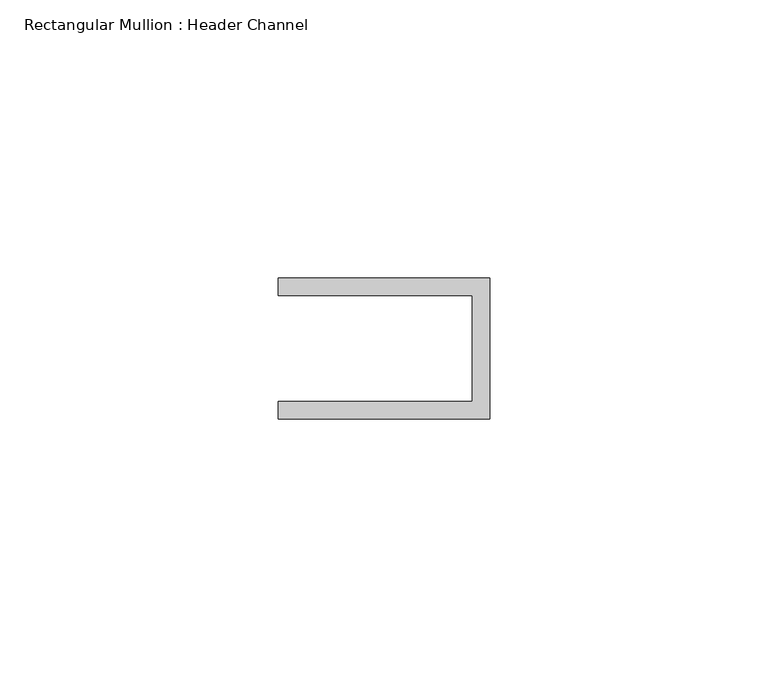
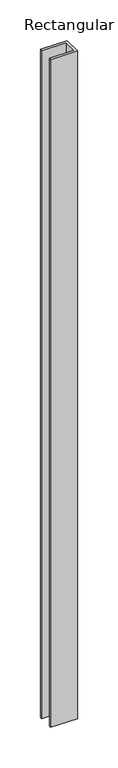
"""IFC4 building model written with IfcOpenShell, lengths in millimetres: member geometry, Rectangular Mullion : Header Channel."""

import ifcopenshell
import ifcopenshell.guid

model = None  # the IFC model being written
_history = None  # IfcOwnerHistory: only IFC2X3 demands one
_inside = {}  # id of a spatial element -> (the spatial element, [elements in it])
_under = {}  # id of a project, library or spatial element -> (it, [spatial elements below it])
_declared = {}  # id of a project -> (the project, [libraries it declares])
_typed = {}  # id of a type object -> (the type object, [elements of that type])
_made_of = {}  # id of a material, layer set ... -> (it, [elements and type objects made of it])


def new_model(schema):
    """Start an empty IFC model of exactly this schema.

    Asked for "IFC4X3", IfcOpenShell would pick the latest addendum, in which some entities
    have other attributes; the version numbers below select the first issue.
    IFC2X3 requires an IfcOwnerHistory on every rooted entity: one is made here for all.
    """
    global model, _history
    if schema == "IFC4X3":
        model = ifcopenshell.file(schema_version=(4, 3, 0, 0))
    else:
        model = ifcopenshell.file(schema=schema)
    _inside.clear()
    _under.clear()
    _declared.clear()
    _typed.clear()
    _made_of.clear()
    _history = None
    if model.schema == "IFC2X3":
        org = make("IfcOrganization", Name="unknown")
        user = make(
            "IfcPersonAndOrganization",
            ThePerson=make("IfcPerson", FamilyName="unknown"),
            TheOrganization=org,
        )
        app = make(
            "IfcApplication",
            ApplicationDeveloper=org,
            Version="unknown",
            ApplicationFullName="unknown",
            ApplicationIdentifier="unknown",
        )
        _history = make(
            "IfcOwnerHistory",
            OwningUser=user,
            OwningApplication=app,
            ChangeAction="ADDED",
            CreationDate=0,
        )
    return model


def make(cls, **values):
    """One entity of the class cls with the attributes given. An attribute that is None is left unset."""
    return model.create_entity(
        cls, **{name: value for name, value in values.items() if value is not None}
    )


def rooted(cls, **values):
    """An entity with a GlobalId (a new one), such as an element, a storey or a relation."""
    return make(cls, GlobalId=ifcopenshell.guid.new(), OwnerHistory=_history, **values)


def si_unit(unit_type, name, prefix=None):
    """IfcSIUnit, for example si_unit("LENGTHUNIT", "METRE", prefix="MILLI")."""
    return make("IfcSIUnit", UnitType=unit_type, Prefix=prefix, Name=name)


def assignment(units):
    """IfcUnitAssignment: the units of a project."""
    return None if units is None else make("IfcUnitAssignment", Units=units)


def point(xyz):
    """IfcCartesianPoint."""
    return None if xyz is None else make("IfcCartesianPoint", Coordinates=xyz)


def direction(xyz):
    """IfcDirection."""
    return None if xyz is None else make("IfcDirection", DirectionRatios=xyz)


def frame(location, z_axis=None, x_axis=None):
    """IfcAxis2Placement3D, a coordinate frame: its origin and axes. An axis left out is left unset."""
    return make(
        "IfcAxis2Placement3D",
        Location=point(location),
        Axis=direction(z_axis),
        RefDirection=direction(x_axis),
    )


def origin():
    """The frame at (0, 0, 0) with its axes left unset."""
    return frame((0.0, 0.0, 0.0))


def place(relative_to, where):
    """IfcLocalPlacement: puts the frame where relative to a parent placement (None: the world)."""
    return make(
        "IfcLocalPlacement", PlacementRelTo=relative_to, RelativePlacement=where
    )


def context(
    kind, dimensions, precision=None, world=None, true_north=None, identifier=None
):
    """IfcGeometricRepresentationContext, for example the 3D "Model" context."""
    return make(
        "IfcGeometricRepresentationContext",
        ContextIdentifier=identifier,
        ContextType=kind,
        CoordinateSpaceDimension=dimensions,
        Precision=precision,
        WorldCoordinateSystem=world,
        TrueNorth=true_north,
    )


def project(units=None, contexts=None):
    """IfcProject with its units and contexts."""
    return rooted(
        "IfcProject",
        Name="project",
        RepresentationContexts=contexts,
        UnitsInContext=assignment(units),
    )


def spatial(cls, under=None, at=None, **own):
    """A site, building, storey or space (cls), placed at a placement, below another one or the project."""
    s = rooted(cls, ObjectPlacement=at, **own)
    if under is not None:
        _under.setdefault(under.id(), (under, []))[1].append(s)
    return s


def polyline(points):
    """IfcPolyline through the points."""
    return make("IfcPolyline", Points=[point(p) for p in points])


def outline(outer, holes=None, kind="AREA"):
    """IfcArbitraryClosedProfileDef: a profile drawn as a closed curve; with holes, ...WithVoids."""
    if holes is None:
        return make("IfcArbitraryClosedProfileDef", ProfileType=kind, OuterCurve=outer)
    return make(
        "IfcArbitraryProfileDefWithVoids",
        ProfileType=kind,
        OuterCurve=outer,
        InnerCurves=holes,
    )


def extrude(swept, where, along, depth):
    """IfcExtrudedAreaSolid: the profile swept, set in the frame where, extruded along a direction by depth."""
    return make(
        "IfcExtrudedAreaSolid",
        SweptArea=swept,
        Position=where,
        ExtrudedDirection=direction(along),
        Depth=depth,
    )


def shape(context_of_items, identifier, shape_type, items):
    """IfcShapeRepresentation: the items that make up one representation, for example the "Body"."""
    return make(
        "IfcShapeRepresentation",
        ContextOfItems=context_of_items,
        RepresentationIdentifier=identifier,
        RepresentationType=shape_type,
        Items=items,
    )


def source(mapping_origin, context_of_items, identifier, shape_type, items):
    """IfcRepresentationMap: a shape defined once, which mapped items show again and again."""
    return make(
        "IfcRepresentationMap",
        MappingOrigin=mapping_origin,
        MappedRepresentation=shape(context_of_items, identifier, shape_type, items),
    )


def transform(
    local_origin,
    x_axis=None,
    y_axis=None,
    z_axis=None,
    scale=None,
    scale2=None,
    scale3=None,
    uniform=True,
):
    """IfcCartesianTransformationOperator3D, or its non-uniform kind. x_axis, y_axis, z_axis: its Axis1, 2, 3."""
    if uniform:
        return make(
            "IfcCartesianTransformationOperator3D",
            Axis1=direction(x_axis),
            Axis2=direction(y_axis),
            LocalOrigin=point(local_origin),
            Scale=scale,
            Axis3=direction(z_axis),
        )
    return make(
        "IfcCartesianTransformationOperator3DnonUniform",
        Axis1=direction(x_axis),
        Axis2=direction(y_axis),
        LocalOrigin=point(local_origin),
        Scale=scale,
        Axis3=direction(z_axis),
        Scale2=scale2,
        Scale3=scale3,
    )


def mapped(mapping_source, mapping_target):
    """IfcMappedItem: shows the shape of a source again, moved by a transform."""
    return make(
        "IfcMappedItem", MappingSource=mapping_source, MappingTarget=mapping_target
    )


def made_of(thing, what):
    """Note that an element or type object is made of a material, layer set ...; save() writes the relation."""
    if what is not None:
        _made_of.setdefault(what.id(), (what, []))[1].append(thing)
    return thing


def element(
    cls,
    number,
    at=None,
    inside=None,
    cuts=None,
    type_object=None,
    material=None,
    context=None,
    identifier="Body",
    shape_type=None,
    held_by="IfcProductDefinitionShape",
    body=None,
    shapes=None,
    **own,
):
    """One element of the class cls, such as IfcWall. Its Tag is "e" and its number.

    at: its placement. inside: the storey or other place that contains it. cuts: it is an
    opening in that element (IfcRelVoidsElement). A single representation is given by context,
    identifier, shape_type and body (its items); several are given by shapes. held_by: the class
    of the entity that holds the representations. save() writes the other relations.
    """
    e = rooted(cls, Tag="e%d" % number, ObjectPlacement=at, **own)
    if body is not None:
        shapes = [shape(context, identifier, shape_type, body)]
    if shapes is not None:
        e.Representation = make(held_by, Representations=shapes)
    if inside is not None:
        _inside.setdefault(inside.id(), (inside, []))[1].append(e)
    if cuts is not None:
        rooted(
            "IfcRelVoidsElement", RelatingBuildingElement=cuts, RelatedOpeningElement=e
        )
    if type_object is not None:
        _typed.setdefault(type_object.id(), (type_object, []))[1].append(e)
    return made_of(e, material)


def aggregate(whole, parts):
    """IfcRelAggregates: a whole, such as a stair, and the parts it consists of."""
    return rooted("IfcRelAggregates", RelatingObject=whole, RelatedObjects=parts)


def save(model, path):
    """Write the relations noted so far, then the file.

    IfcRelAggregates (storeys below a building ...), IfcRelContainedInSpatialStructure (elements
    in a storey), IfcRelDefinesByType, IfcRelAssociatesMaterial and IfcRelDeclares: one each for
    every whole, place, type object, material and project.
    """
    for whole, parts in _under.values():
        aggregate(whole, parts)
    for where, things in _inside.values():
        rooted(
            "IfcRelContainedInSpatialStructure",
            RelatedElements=things,
            RelatingStructure=where,
        )
    for kind, things in _typed.values():
        rooted("IfcRelDefinesByType", RelatedObjects=things, RelatingType=kind)
    for what, things in _made_of.values():
        rooted("IfcRelAssociatesMaterial", RelatedObjects=things, RelatingMaterial=what)
    for by, libraries in _declared.values():
        rooted("IfcRelDeclares", RelatingContext=by, RelatedDefinitions=libraries)
    model.write(path)


def rectangular_mullion_header_channel_9847aa58(model_context):
    return source(origin(), model_context, "Body", "SweptSolid", [
        extrude(outline(polyline([(0.0, -12.7), (-38.1, -12.7), (-38.1, -9.525), (-3.175, -9.525), (-3.175, 9.525), (-38.1, 9.525), (-38.1, 12.7), (0.0, 12.7), (0.0, -12.7)])), frame((0.0, 0.0, -1005.4166667), z_axis=(0.0, 0.0, 1.0), x_axis=(1.0, 0.0, 0.0)), (0.0, 0.0, 1.0), 1005.4166667),
    ])


if __name__ == "__main__":
    model = new_model("IFC4")
    model_context = context("Model", 3, world=origin())
    ifc_project = project(units=[si_unit("LENGTHUNIT", "METRE", prefix="MILLI")], contexts=[model_context])
    site = spatial("IfcSite", under=ifc_project)
    building = spatial("IfcBuilding", under=site)
    placement = place(None, origin())
    rectangular_mullion_header_channel_shape = rectangular_mullion_header_channel_9847aa58(model_context)
    element("IfcMember", 1, ObjectType="Rectangular Mullion : Header Channel", at=placement, inside=building, context=model_context, shape_type="MappedRepresentation", body=[
        mapped(rectangular_mullion_header_channel_shape, transform((0.0, 0.0, 0.0), x_axis=(1.0, 0.0, 0.0), y_axis=(0.0, 1.0, 0.0), z_axis=(0.0, 0.0, 1.0))),
    ])
    save(model, "model.ifc")

# Revit data of these elements
# Type "Rectangular Mullion : Header Channel"
#   built-in parameter 1007322 = 0.0833333 (stored number, unit not read)
#   built-in parameter 1007321 = -0.03125 (stored number, unit not read)
#   built-in parameter 1007320 = 0.0416667 (stored number, unit not read)
# Element 1 (IfcMember, "Rectangular Mullion : Header Channel")
#   Materials on its faces: "ALUM"
# Materials
#   "ALUM": class "Generic", colour RGB 157 157 157, transparency 0, Cost = 0
